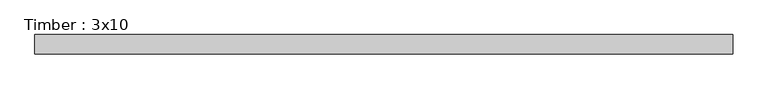
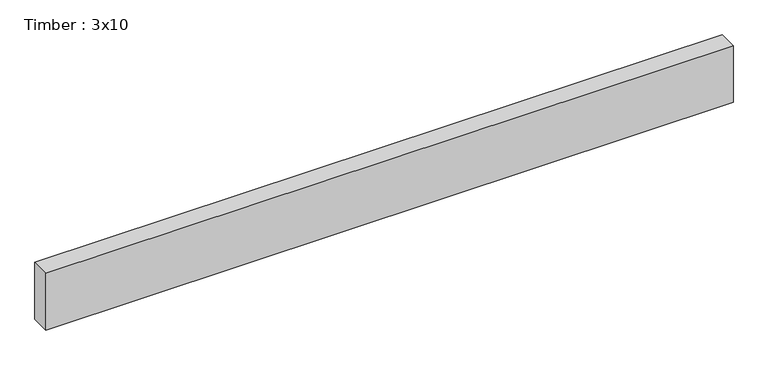
"""IFC4 building model written with IfcOpenShell, lengths in millimetres: beam geometry, Timber : 3x10."""

from ifc_helpers import new_model, si_unit, frame, origin, place, context, project, spatial, polyline, outline, extrude, source, transform, mapped, element, save


def timber_3x10_6eb33a06(model_context):
    return source(origin(), model_context, "Body", "SweptSolid", [
        extrude(outline(polyline([(1384.3, 38.1), (1384.3, -38.1), (-1384.2999994, -38.1), (-1384.2999994, 38.1), (1384.3, 38.1)])), frame((0.0, 0.0, -120.65), z_axis=(0.0, 0.0, 1.0), x_axis=(1.0, 0.0, 0.0)), (0.0, 0.0, 1.0), 241.3),
    ])


if __name__ == "__main__":
    model = new_model("IFC4")
    model_context = context("Model", 3, world=origin())
    ifc_project = project(units=[si_unit("LENGTHUNIT", "METRE", prefix="MILLI")], contexts=[model_context])
    site = spatial("IfcSite", under=ifc_project)
    building = spatial("IfcBuilding", under=site)
    placement = place(None, origin())
    timber_3x10_shape = timber_3x10_6eb33a06(model_context)
    element("IfcBeam", 1, ObjectType="Timber : 3x10", at=placement, inside=building, context=model_context, shape_type="MappedRepresentation", body=[
        mapped(timber_3x10_shape, transform((0.0, 0.0, 0.0), x_axis=(1.0, 0.0, 0.0), y_axis=(0.0, 1.0, 0.0), z_axis=(0.0, 0.0, 1.0))),
    ])
    save(model, "model.ifc")

# Revit data of these elements
# Type "Timber : 3x10"
#   Assembly Code = "B10"
#   A = 0.362847 SF
#   Length [instance default] = 5' - 0"
#   b = 0' - 3"
#   d = 0' - 9 1/2"
#   Structural Material [instance default] = Softwood, Lumber
# Element 1 (IfcBeam, "Timber : 3x10")
#   Materials on its faces: "Softwood, Lumber"
# Materials
#   "Softwood, Lumber": class "Wood", colour RGB 144 113 62, transparency 0, Description = "Pinus Echinata", Cost = 0
